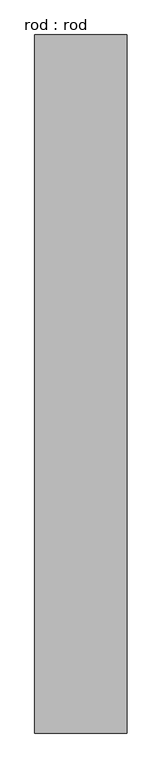
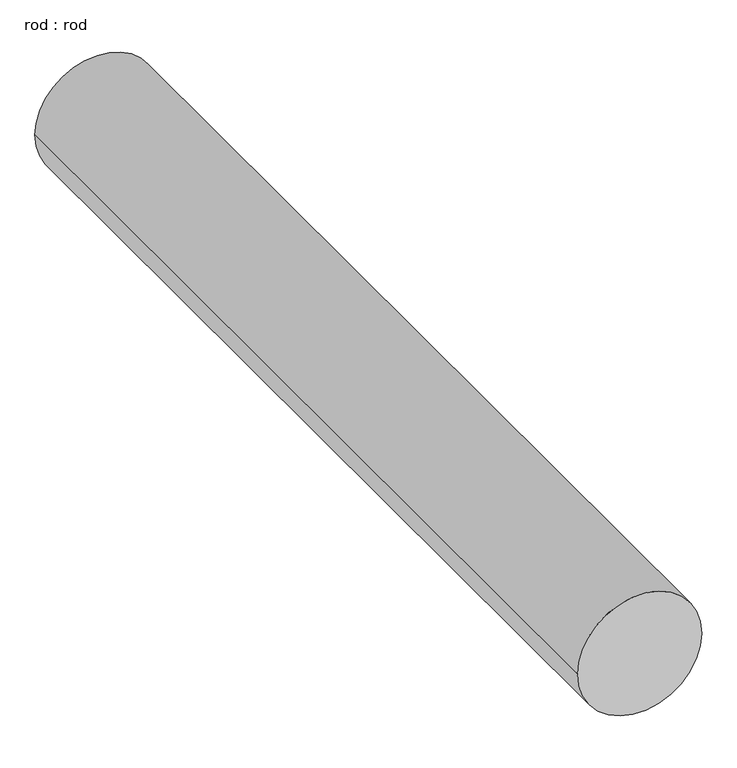
"""IFC4 building model written with IfcOpenShell, lengths in millimetres: proxy geometry, rod : rod."""

from ifc_helpers import new_model, si_unit, point, frame, frame_2d, origin, place, context, project, spatial, circle_curve, trimmed, segment, composite_curve, outline, extrude, source, transform, mapped, element, save


def rod_rod_cd5573c2(model_context):
    return source(origin(), model_context, "Body", "SweptSolid", [
        extrude(outline(composite_curve([segment(trimmed(circle_curve(frame_2d((0.0108462, 0.0)), 200.0), [point((0.0108462, 200.0))], [point((0.0108462, -200.0))], False, "CARTESIAN"), True, "CONTINUOUS"), segment(trimmed(circle_curve(frame_2d((0.0108462, 0.0)), 200.0), [point((0.0108462, -200.0))], [point((0.0108462, 200.0))], False, "CARTESIAN"), True, "CONTINUOUS")], self_intersect=False)), frame((0.0, 2582.0143296, 0.0), z_axis=(0.0, 1.0, 0.0), x_axis=(0.0, 0.0, 1.0)), (0.0, 0.0, 1.0), 3021.4285714),
    ])


if __name__ == "__main__":
    model = new_model("IFC4")
    model_context = context("Model", 3, world=origin())
    ifc_project = project(units=[si_unit("LENGTHUNIT", "METRE", prefix="MILLI")], contexts=[model_context])
    site = spatial("IfcSite", under=ifc_project)
    building = spatial("IfcBuilding", under=site)
    placement = place(None, origin())
    rod_rod_shape = rod_rod_cd5573c2(model_context)
    element("IfcBuildingElementProxy", 1, Name="rod : rod", ObjectType="rod : rod", at=placement, inside=building, context=model_context, shape_type="MappedRepresentation", body=[
        mapped(rod_rod_shape, transform((0.0, 0.0, 0.0), x_axis=(1.0, 0.0, 0.0), y_axis=(0.0, 1.0, 0.0), z_axis=(0.0, 0.0, 1.0))),
    ])
    save(model, "model.ifc")

# Revit data of these elements
# Type "rod : rod"
#   Default Elevation = 0
